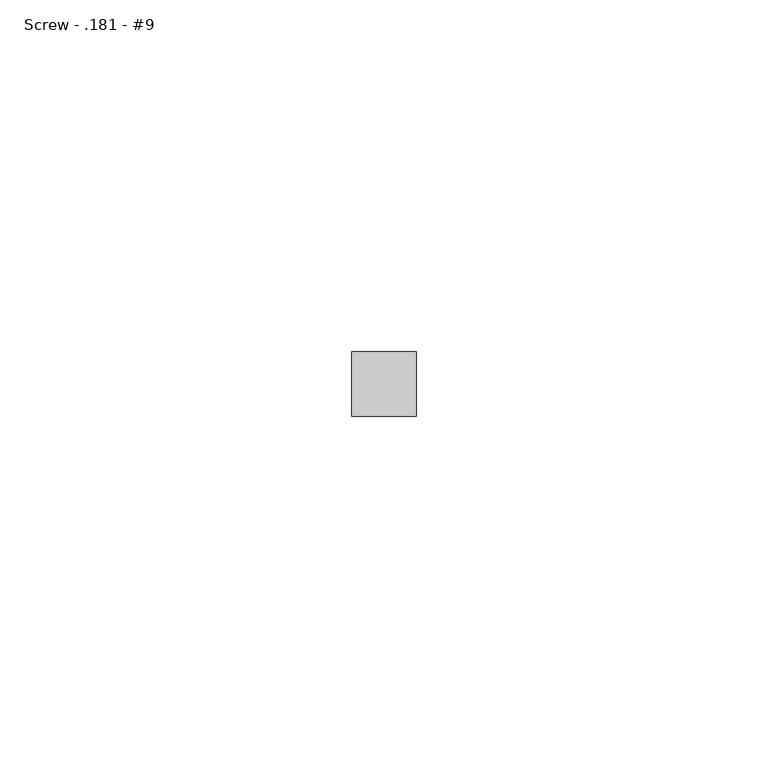
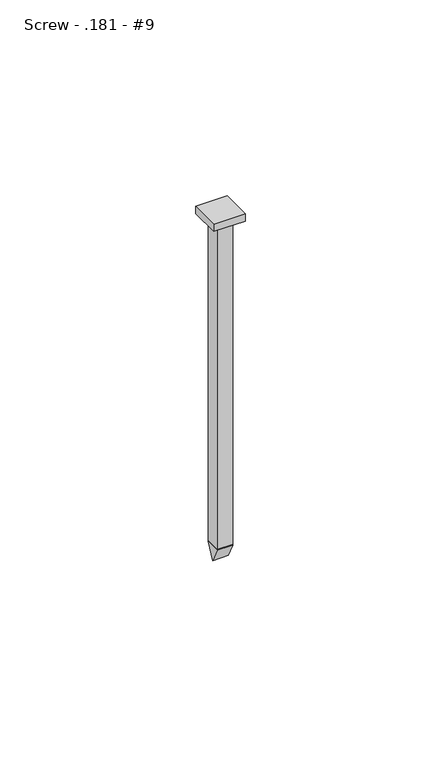
"""IFC4 building model written with IfcOpenShell, lengths in millimetres: fastener geometry, 060523 - W_P_C - Fastenings - Generic - SQUARE : Screw - .181 - #9."""

from ifc_helpers import new_model, si_unit, frame, origin, origin_with_axes, place, context, project, spatial, polyline, outline, extrude, source, transform, mapped, element, save


def screw_181_9_f4ff6ace(model_context):
    return source(origin(), model_context, "Body", "SweptSolid", [
        extrude(outline(polyline([(0.0, -106.1974), (-2.2987, -101.6), (2.2987, -101.6), (0.0, -106.1974)])), frame((-2.2987, 0.0, 0.0), z_axis=(1.0, 0.0, 0.0), x_axis=(0.0, 1.0, 0.0)), (0.0, 0.0, 1.0), 4.5974),
        extrude(outline(polyline([(-4.5974, -4.5974), (-4.5974, 4.5974), (4.5974, 4.5974), (4.5974, -4.5974), (-4.5974, -4.5974)])), origin_with_axes(), (0.0, 0.0, 1.0), 2.2987),
        extrude(outline(polyline([(-2.2987, 2.2987), (2.2987, 2.2987), (2.2987, -2.2987), (-2.2987, -2.2987), (-2.2987, 2.2987)])), frame((0.0, 0.0, -101.6), z_axis=(0.0, 0.0, 1.0), x_axis=(1.0, 0.0, 0.0)), (0.0, 0.0, 1.0), 101.6),
    ])


if __name__ == "__main__":
    model = new_model("IFC4")
    model_context = context("Model", 3, world=origin())
    ifc_project = project(units=[si_unit("LENGTHUNIT", "METRE", prefix="MILLI")], contexts=[model_context])
    site = spatial("IfcSite", under=ifc_project)
    building = spatial("IfcBuilding", under=site)
    placement = place(None, origin())
    screw_181_9_shape = screw_181_9_f4ff6ace(model_context)
    element("IfcFastener", 1, ObjectType="060523 - W_P_C - Fastenings - Generic - SQUARE : Screw - .181 - #9", at=placement, inside=building, context=model_context, shape_type="MappedRepresentation", body=[
        mapped(screw_181_9_shape, transform((0.0, 0.0, 0.0), x_axis=(1.0, 0.0, 0.0), y_axis=(0.0, 1.0, 0.0), z_axis=(0.0, 0.0, 1.0))),
    ])
    save(model, "model.ifc")

# Revit data of these elements
# Type "060523 - W_P_C - Fastenings - Generic - SQUARE : Screw - .181 - #9"
#   Washer_Thickness = 0' - 0.00333"
#   Washer Radius = 0' - 0.1005"
#   Washer Offset - Head = 0' - 0"
#   Washer Offset = 0' - 0"
#   Thickness_of_Substrate [instance default] = 0' - 1"
#   Side = 0' - 0 37/64"
#   Radius = 0' - 0.0905"
#   Length [instance default] = 0' - 4"
#   Head Size = 0' - 1"
#   Head Radius = 0' - 0 1/2"
#   Head Height = 0' - 0.01"
#   Double Diameter = 0' - 0.362"
#   Diameter = 0' - 0.181"
#   Default Elevation = 4' - 0"
#   Washer_Nut_Visibility = no
#   Washer_Head_Visibility = no
#   Round_Head_Visibility = yes
#   Point Visibility = yes
#   Nut_Visibility = no
#   Hex_Head_Visiblilty = no
#   Washer Material = none
#   Bolt Material (Size) = AT SILL - FASTENER AT 24" O.C.
# Materials
#   "AT SILL - FASTENER AT 24\" O.C.": class "Generic", colour RGB 120 120 120, transparency 0, Cost = 0
